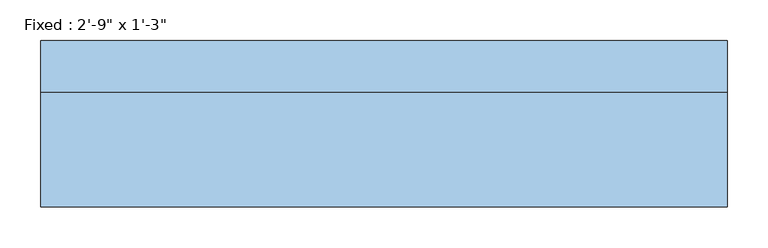
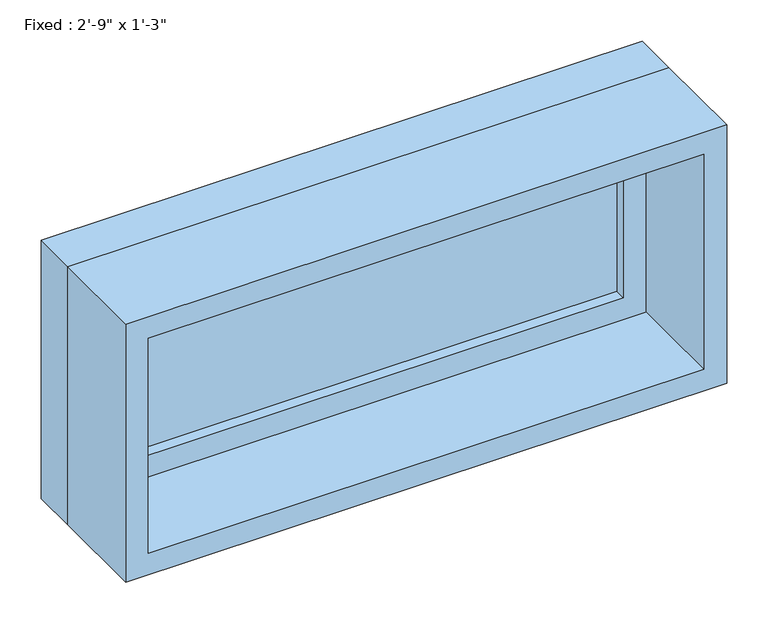
"""IFC4 building model written with IfcOpenShell, lengths in millimetres: window geometry."""

from ifc_helpers import new_model, si_unit, frame, origin, place, context, project, spatial, polyline, outline, extrude, source, transform, mapped, element, save


def window_df5485c9(model_context):
    return source(origin(), model_context, "Body", "SweptSolid", [
        extrude(outline(polyline([(317.5, 53.975), (-393.7, 53.975), (-393.7, 66.675), (317.5, 66.675), (317.5, 53.975)])), frame((0.0, 0.0, 977.9), z_axis=(0.0, 0.0, 1.0), x_axis=(1.0, 0.0, 0.0)), (0.0, 0.0, 1.0), 254.0),
        extrude(outline(polyline([(1276.35, -438.15), (933.45, -438.15), (933.45, 361.95), (1276.35, 361.95), (1276.35, -438.15)]), holes=[polyline([(1231.9, -393.7), (1231.9, 317.5), (977.9, 317.5), (977.9, -393.7), (1231.9, -393.7)])]), frame((0.0, 38.1, 0.0), z_axis=(0.0, 1.0, 0.0), x_axis=(0.0, 0.0, 1.0)), (0.0, 0.0, 1.0), 44.45),
        extrude(outline(polyline([(1295.4, -457.2), (914.4, -457.2), (914.4, 381.0), (1295.4, 381.0), (1295.4, -457.2)]), holes=[polyline([(1263.65, -425.45), (1263.65, 349.25), (946.15, 349.25), (946.15, -425.45), (1263.65, -425.45)])]), frame((0.0, -101.6, 0.0), z_axis=(0.0, 1.0, 0.0), x_axis=(0.0, 0.0, 1.0)), (0.0, 0.0, 1.0), 139.7),
        extrude(outline(polyline([(1295.4, 381.0), (1295.4, -457.2), (914.4, -457.2), (914.4, 381.0), (1295.4, 381.0)]), holes=[polyline([(1276.35, 361.95), (933.45, 361.95), (933.45, -438.15), (1276.35, -438.15), (1276.35, 361.95)])]), frame((0.0, 38.1, 0.0), z_axis=(0.0, 1.0, 0.0), x_axis=(0.0, 0.0, 1.0)), (0.0, 0.0, 1.0), 63.5),
    ])


if __name__ == "__main__":
    model = new_model("IFC4")
    model_context = context("Model", 3, world=origin())
    ifc_project = project(units=[si_unit("LENGTHUNIT", "METRE", prefix="MILLI")], contexts=[model_context])
    site = spatial("IfcSite", under=ifc_project)
    building = spatial("IfcBuilding", under=site)
    placement = place(None, origin())
    window_shape = window_df5485c9(model_context)
    element("IfcWindow", 1, ObjectType="Fixed : 2'-9\" x 1'-3\"", at=placement, inside=building, context=model_context, shape_type="MappedRepresentation", body=[
        mapped(window_shape, transform((0.0, 0.0, 0.0), x_axis=(1.0, 0.0, 0.0), y_axis=(0.0, 1.0, 0.0), z_axis=(0.0, 0.0, 1.0))),
    ])
    save(model, "model.ifc")

# Revit data of these elements
# Type "Fixed : 2'-9\" x 1'-3\""
#   Type Mark = "29"
#   Construction Type Id = "GSP4R"
#   Assembly Code = "B2020100"
#   Analytic Construction = "1/8 in Pilkington single glazing"
#   Visual Light Transmittance = 0.9
#   Solar Heat Gain Coefficient = 0.78
#   Heat Transfer Coefficient (U) = 3.6886 W/(m²·K)
#   Height = 1' - 3"
#   Default Sill Height = 3' - 0"
#   Width = 2' - 9"
#   Window Inset = 0' - 0 3/4"
#   Glass Pane Material = Glass
#   Sash Material = Sash
#   Wall Closure = (empty or 0)
# Element 1 (IfcWindow, "Fixed : 2'-9\" x 1'-3\"")
#   Materials on its faces: "Sash", "Glass"
# Materials
#   "Glass": class "Glass", colour RGB 0 128 192, transparency 0.75, Description = "Soda Lime Glass", Cost = 0
#   "Sash": class "Wood", colour RGB 224 178 126, transparency 0, Cost = 0
